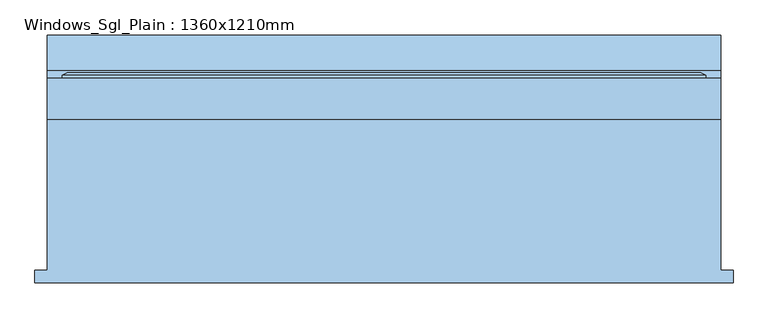
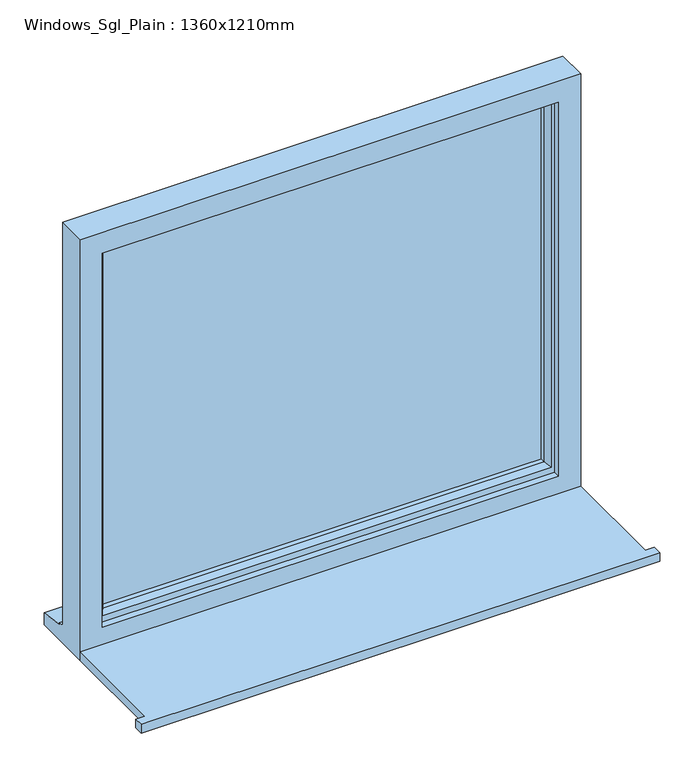
"""IFC4 building model written with IfcOpenShell, lengths in millimetres: window geometry, Windows_Sgl_Plain : 1360x1210mm."""

from ifc_helpers import new_model, si_unit, frame, origin, place, context, project, spatial, polyline, outline, extrude, faceted_brep, source, transform, mapped, element, save


def windows_sgl_plain_1360x1210mm_d7fcc91f(model_context):
    return source(origin(), model_context, "Body", "SolidModel", [
        extrude(outline(polyline([(-705.0, -235.2934322), (-705.0, -210.2934322), (-680.0, -210.2934322), (-680.0, 94.2065678), (680.0, 94.2065678), (680.0, -210.2934322), (705.0, -210.2934322), (705.0, -235.2934322), (-705.0, -235.2934322)])), frame((0.0, 0.0, 900.0), z_axis=(0.0, 0.0, 1.0), x_axis=(1.0, 0.0, 0.0)), (0.0, 0.0, 1.0), 25.0),
        faceted_brep([(-680.0, 94.2065678, 900.0), (680.0, 94.2065678, 900.0), (680.0, 94.2065678, 2110.0), (-680.0, 94.2065678, 2110.0), (-620.0, 94.2065678, 2050.0), (620.0, 94.2065678, 2050.0), (620.0, 94.2065678, 975.0), (-620.0, 94.2065678, 975.0), (-680.0, 177.2065678, 2110.0), (-680.0, 177.2065678, 951.0), (-680.0, 192.2065678, 949.68767), (-680.0, 192.2065678, 944.7449676), (-680.0, 264.7065678, 933.8088847), (-680.0, 264.7065678, 900.0), (680.0, 177.2065678, 2110.0), (680.0, 177.2065678, 951.0), (-640.0, 177.2065678, 2070.0), (-640.0, 177.2065678, 963.0), (640.0, 177.2065678, 963.0), (640.0, 177.2065678, 2070.0), (-640.0, 112.2065678, 2070.0), (-640.0, 112.2065678, 963.0), (640.0, 112.2065678, 2070.0), (640.0, 112.2065678, 963.0), (-620.0, 112.2065678, 2050.0), (-620.0, 112.2065678, 975.0), (620.0, 112.2065678, 975.0), (620.0, 112.2065678, 2050.0), (680.0, 264.7065678, 900.0), (680.0, 264.7065678, 933.8088847), (680.0, 192.2065678, 944.7449676), (680.0, 192.2065678, 949.68767)], [[[0, 1, 2, 3], [4, 5, 6, 7]], [[0, 3, 8, 9, 10, 11, 12, 13]], [[9, 8, 14, 15], [16, 17, 18, 19]], [[17, 16, 20, 21]], [[20, 22, 23, 21], [24, 25, 26, 27]], [[24, 4, 7, 25]], [[3, 2, 14, 8]], [[16, 19, 22, 20]], [[5, 4, 24, 27]], [[15, 14, 2, 1, 28, 29, 30, 31]], [[19, 18, 23, 22]], [[5, 27, 26, 6]], [[28, 1, 0, 13]], [[29, 28, 13, 12]], [[30, 29, 12, 11]], [[31, 30, 11, 10]], [[15, 31, 10, 9]], [[21, 23, 18, 17]], [[7, 6, 26, 25]]]),
        extrude(outline(polyline([(610.0, 141.2065678), (-610.0, 141.2065678), (-610.0, 165.2065678), (610.0, 165.2065678), (610.0, 141.2065678)])), frame((0.0, 0.0, 993.0), z_axis=(0.0, 0.0, 1.0), x_axis=(1.0, 0.0, 0.0)), (0.0, 0.0, 1.0), 1047.0),
        faceted_brep([(-650.0, 177.2065678, 2080.0), (-650.0, 182.9800705, 2080.0), (-650.0, 182.9800705, 953.0), (-650.0, 177.2065678, 953.0), (-640.0, 112.2065678, 2070.0), (-640.0, 177.2065678, 2070.0), (-640.0, 177.2065678, 963.0), (-640.0, 112.2065678, 963.0), (-600.0, 126.6994677, 2030.0), (-610.1480377, 112.2065678, 2040.1480377), (-610.1480377, 112.2065678, 992.8519623), (-600.0, 126.6994677, 1003.0), (-600.0, 141.2065678, 2030.0), (-600.0, 141.2065678, 1003.0), (-610.0, 165.2065678, 2040.0), (-610.0, 141.2065678, 2040.0), (-610.0, 141.2065678, 993.0), (-610.0, 165.2065678, 993.0), (-600.0, 182.9800705, 2030.0), (-600.0, 165.2065678, 2030.0), (-600.0, 165.2065678, 1003.0), (-600.0, 182.9800705, 1003.0), (-617.4457548, 188.7535732, 2047.4457548), (-617.4457548, 188.7535732, 985.5542452), (-639.2153903, 188.7535732, 2069.2153903), (-639.2153903, 188.7535732, 963.7846097), (650.0, 182.9800705, 953.0), (650.0, 177.2065678, 953.0), (640.0, 177.2065678, 963.0), (640.0, 112.2065678, 963.0), (610.1480377, 112.2065678, 992.8519623), (600.0, 126.6994677, 1003.0), (600.0, 141.2065678, 1003.0), (610.0, 141.2065678, 993.0), (610.0, 165.2065678, 993.0), (600.0, 165.2065678, 1003.0), (600.0, 182.9800705, 1003.0), (617.4457548, 188.7535732, 985.5542452), (639.2153903, 188.7535732, 963.7846097), (650.0, 182.9800705, 2080.0), (650.0, 177.2065678, 2080.0), (640.0, 177.2065678, 2070.0), (640.0, 112.2065678, 2070.0), (610.1480377, 112.2065678, 2040.1480377), (600.0, 126.6994677, 2030.0), (600.0, 141.2065678, 2030.0), (610.0, 141.2065678, 2040.0), (610.0, 165.2065678, 2040.0), (600.0, 165.2065678, 2030.0), (600.0, 182.9800705, 2030.0), (617.4457548, 188.7535732, 2047.4457548), (639.2153903, 188.7535732, 2069.2153903)], [[[0, 1, 2, 3]], [[4, 5, 6, 7]], [[8, 9, 10, 11]], [[12, 8, 11, 13]], [[14, 15, 16, 17]], [[18, 19, 20, 21]], [[22, 18, 21, 23]], [[1, 24, 25, 2]], [[3, 2, 26, 27]], [[7, 6, 28, 29]], [[11, 10, 30, 31]], [[13, 11, 31, 32]], [[17, 16, 33, 34]], [[21, 20, 35, 36]], [[23, 21, 36, 37]], [[2, 25, 38, 26]], [[27, 26, 39, 40]], [[29, 28, 41, 42]], [[31, 30, 43, 44]], [[32, 31, 44, 45]], [[34, 33, 46, 47]], [[36, 35, 48, 49]], [[37, 36, 49, 50]], [[26, 38, 51, 39]], [[40, 39, 1, 0]], [[3, 27, 40, 0], [5, 41, 28, 6]], [[42, 41, 5, 4]], [[7, 29, 42, 4], [9, 43, 30, 10]], [[44, 43, 9, 8]], [[45, 44, 8, 12]], [[15, 46, 33, 16], [13, 32, 45, 12]], [[47, 46, 15, 14]], [[17, 34, 47, 14], [19, 48, 35, 20]], [[49, 48, 19, 18]], [[50, 49, 18, 22]], [[24, 51, 38, 25], [23, 37, 50, 22]], [[39, 51, 24, 1]]]),
    ])


if __name__ == "__main__":
    model = new_model("IFC4")
    model_context = context("Model", 3, world=origin())
    ifc_project = project(units=[si_unit("LENGTHUNIT", "METRE", prefix="MILLI")], contexts=[model_context])
    site = spatial("IfcSite", under=ifc_project)
    building = spatial("IfcBuilding", under=site)
    placement = place(None, origin())
    windows_sgl_plain_1360x1210mm_shape = windows_sgl_plain_1360x1210mm_d7fcc91f(model_context)
    element("IfcWindow", 1, ObjectType="Windows_Sgl_Plain : 1360x1210mm", at=placement, inside=building, context=model_context, shape_type="MappedRepresentation", body=[
        mapped(windows_sgl_plain_1360x1210mm_shape, transform((0.0, 0.0, 0.0), x_axis=(1.0, 0.0, 0.0), y_axis=(0.0, 1.0, 0.0), z_axis=(0.0, 0.0, 1.0))),
    ])
    save(model, "model.ifc")

# Revit data of these elements
# Type "Windows_Sgl_Plain : 1360x1210mm"
#   Type Mark = "47"
#   Operation = "SinglePanel"
#   Construction Type Id = "SGL"
#   Manufacturer = "Revit"
#   Keynote = "L10"
#   Analytic Construction = "Large single-glazed windows"
#   Wrap Layers (Ext) from Ext = 102.5 mm
#   Wrap Layers (Int) from Ext = 177.5 mm
#   Window Board Projection = 25 mm
#   Window Board Extension = 25 mm
#   Visual Light Transmittance = 0.9
#   Solar Heat Gain Coefficient = 0.86
#   Rough Width = 1360 mm
#   Rough Height = 1210 mm
#   Height = 1210 mm
#   Width = 1360 mm
#   Heat Transfer Coefficient (U) = 5.5617 W/(m²·K)
#   Glazing Thickness = 24 mm
#   FrameOffset - External = 50 mm
#   Frame Depth = 65 mm
#   Default Head Height = 2110 mm
#   Cill Depth = 87.5 mm
#   Cavity Closer Width = 50 mm
#   Cavity Closer Offset from Ext = 102.5 mm
#   Cavity Closer Depth = 85 mm
#   Vis - Cavity Closers = yes
#   Material Trim = Window Frame
#   Material Glass = Glass
#   Material Frame = Window Frame
#   Wall Closure = (empty or 0)
# Element 1 (IfcWindow, "Windows_Sgl_Plain : 1360x1210mm")
#   Materials on its faces: "Window Frame", "Glass"
# Materials
#   "Window Frame": class "Miscellaneous", colour RGB 249 249 249, transparency 0, Keynote = "L10"
#   "Glass": class "Glass", colour RGB 0 128 192, transparency 0.9, Description = "Soda Lime Glass", Cost = 0
